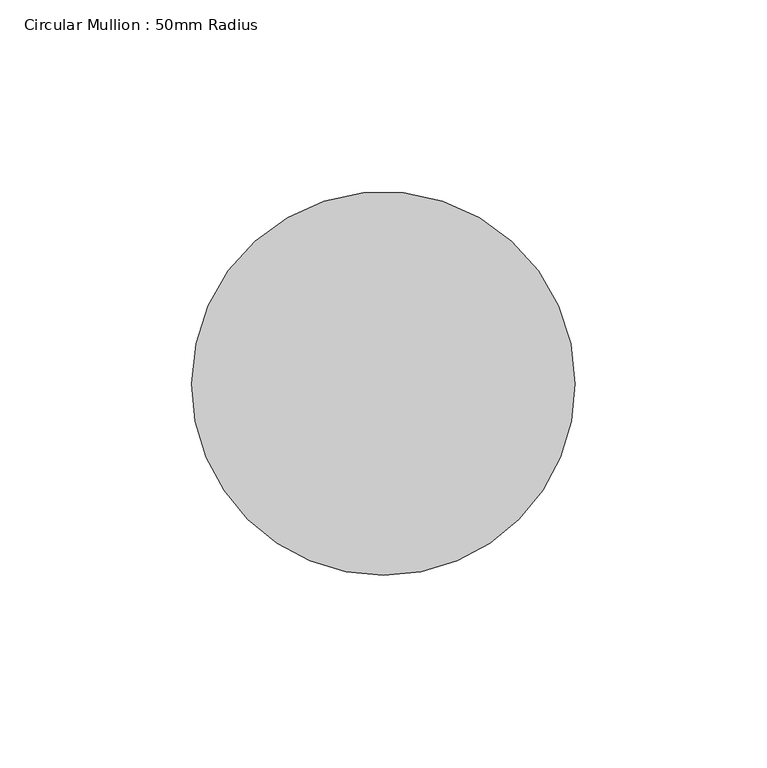
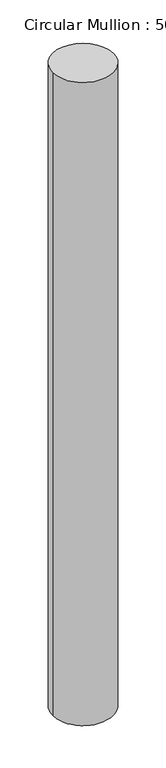
"""IFC4 building model written with IfcOpenShell, lengths in millimetres: member geometry, Circular Mullion : 50mm Radius."""

from ifc_helpers import new_model, si_unit, frame, origin, place, context, project, spatial, ellipse_curve, source, transform, mapped, element, save
from ifc_brep_helpers import plane_surface, cylinder_surface, advanced_brep


def circular_mullion_50mm_radius_0615fb86(model_context):
    return source(origin(), model_context, "Body", "AdvancedBrep", [
        advanced_brep(
        [(-100.0, 0.0, 0.9810349), (0.0, 0.0, 0.0), (0.0, 0.0, -1118.1064768), (-100.0, 0.0, -1119.0505446)],
        [
            (0, 1, ellipse_curve(frame((-50.0, 0.0, 0.4905175), z_axis=(-0.009808851879215107, -0.01445730887826454, -0.9998473746751602), x_axis=(-0.5613583154462035, -0.8273884301367833, 0.017470757144149893)), 50.0076324, 50.0)),
            (1, 2),
            (2, 3, ellipse_curve(frame((-50.0, 0.0, -1118.5785107), z_axis=(-0.009439342938146715, -0.013912688064320377, 0.9998586579690758), x_axis=(0.5613646503839679, 0.8273977672286812, 0.01681261681828095)), 50.0070681, 50.0)),
            (3, 0),
            (1, 0, ellipse_curve(frame((-50.0, 0.0, 0.4905175), z_axis=(-0.009808851879215107, -0.01445730887826454, -0.9998473746751602), x_axis=(-0.5613583154462035, -0.8273884301367833, 0.017470757144149893)), 50.0076324, 50.0)),
            (3, 2, ellipse_curve(frame((-50.0, 0.0, -1118.5785107), z_axis=(-0.009439342938146715, -0.013912688064320377, 0.9998586579690758), x_axis=(0.5613646503839679, 0.8273977672286812, 0.01681261681828095)), 50.0070681, 50.0)),
        ],
        [
            cylinder_surface(frame((-50.0, 0.0, 0.0), z_axis=(0.0, 0.0, 1.0), x_axis=(1.0, 0.0, 0.0)), 50.0),
            plane_surface(frame((-252.2264897, 171.128133, 0.0), z_axis=(0.009808851879215107, 0.01445730887826454, 0.9998473746751602), x_axis=(0.5613583154462027, 0.8273884301367839, -0.017470757144151722))),
            plane_surface(frame((-252.2264897, 171.128133, -1118.1064768), z_axis=(0.009439342938146713, 0.013912688064320373, -0.9998586579690756), x_axis=(0.5613646503839678, 0.827397767228681, 0.01681261681830115))),
        ],
        [
            (0, [[1, 2, 3, 4]]),
            (0, [[5, -4, 6, -2]]),
            (1, [[-1, -5]]),
            (2, [[-6, -3]]),
        ],
    ),
    ])


if __name__ == "__main__":
    model = new_model("IFC4")
    model_context = context("Model", 3, world=origin())
    ifc_project = project(units=[si_unit("LENGTHUNIT", "METRE", prefix="MILLI")], contexts=[model_context])
    site = spatial("IfcSite", under=ifc_project)
    building = spatial("IfcBuilding", under=site)
    placement = place(None, origin())
    circular_mullion_50mm_radius_shape = circular_mullion_50mm_radius_0615fb86(model_context)
    element("IfcMember", 1, ObjectType="Circular Mullion : 50mm Radius", at=placement, inside=building, context=model_context, shape_type="MappedRepresentation", body=[
        mapped(circular_mullion_50mm_radius_shape, transform((0.0, 0.0, 0.0), x_axis=(1.0, 0.0, 0.0), y_axis=(0.0, 1.0, 0.0), z_axis=(0.0, 0.0, 1.0))),
    ])
    save(model, "model.ifc")

# Revit data of these elements
# Type "Circular Mullion : 50mm Radius"
#   built-in parameter 1007350 = 0.164042 (stored number, unit not read)
# Element 1 (IfcMember, "Circular Mullion : 50mm Radius")
#   Materials on its faces: "Aluminium"
# Materials
#   "Aluminium": class "Metal", colour RGB 247 247 247, transparency 0, Description = "Aluminium 6061", Cost = 0
